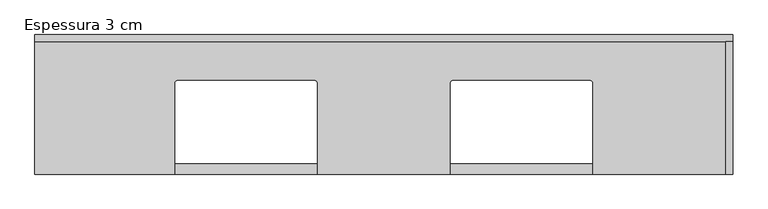
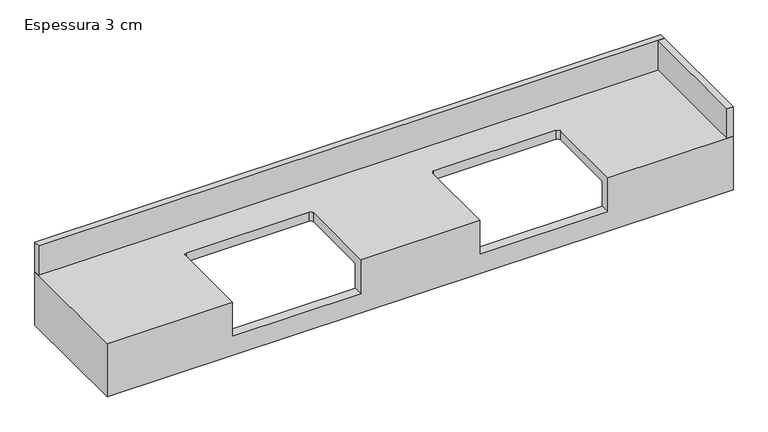
"""IFC4 building model written with IfcOpenShell, lengths in millimetres: furniture geometry, CC_BANCADA BANHEIRO COM DUAS CUBAS_CANTO RETO : Espessura 3 cm."""

import ifcopenshell
import ifcopenshell.guid

model = None  # the IFC model being written
_history = None  # IfcOwnerHistory: only IFC2X3 demands one
_inside = {}  # id of a spatial element -> (the spatial element, [elements in it])
_under = {}  # id of a project, library or spatial element -> (it, [spatial elements below it])
_declared = {}  # id of a project -> (the project, [libraries it declares])
_typed = {}  # id of a type object -> (the type object, [elements of that type])
_made_of = {}  # id of a material, layer set ... -> (it, [elements and type objects made of it])


def new_model(schema):
    """Start an empty IFC model of exactly this schema.

    Asked for "IFC4X3", IfcOpenShell would pick the latest addendum, in which some entities
    have other attributes; the version numbers below select the first issue.
    IFC2X3 requires an IfcOwnerHistory on every rooted entity: one is made here for all.
    """
    global model, _history
    if schema == "IFC4X3":
        model = ifcopenshell.file(schema_version=(4, 3, 0, 0))
    else:
        model = ifcopenshell.file(schema=schema)
    _inside.clear()
    _under.clear()
    _declared.clear()
    _typed.clear()
    _made_of.clear()
    _history = None
    if model.schema == "IFC2X3":
        org = make("IfcOrganization", Name="unknown")
        user = make(
            "IfcPersonAndOrganization",
            ThePerson=make("IfcPerson", FamilyName="unknown"),
            TheOrganization=org,
        )
        app = make(
            "IfcApplication",
            ApplicationDeveloper=org,
            Version="unknown",
            ApplicationFullName="unknown",
            ApplicationIdentifier="unknown",
        )
        _history = make(
            "IfcOwnerHistory",
            OwningUser=user,
            OwningApplication=app,
            ChangeAction="ADDED",
            CreationDate=0,
        )
    return model


def make(cls, **values):
    """One entity of the class cls with the attributes given. An attribute that is None is left unset."""
    return model.create_entity(
        cls, **{name: value for name, value in values.items() if value is not None}
    )


def rooted(cls, **values):
    """An entity with a GlobalId (a new one), such as an element, a storey or a relation."""
    return make(cls, GlobalId=ifcopenshell.guid.new(), OwnerHistory=_history, **values)


def si_unit(unit_type, name, prefix=None):
    """IfcSIUnit, for example si_unit("LENGTHUNIT", "METRE", prefix="MILLI")."""
    return make("IfcSIUnit", UnitType=unit_type, Prefix=prefix, Name=name)


def assignment(units):
    """IfcUnitAssignment: the units of a project."""
    return None if units is None else make("IfcUnitAssignment", Units=units)


def point(xyz):
    """IfcCartesianPoint."""
    return None if xyz is None else make("IfcCartesianPoint", Coordinates=xyz)


def direction(xyz):
    """IfcDirection."""
    return None if xyz is None else make("IfcDirection", DirectionRatios=xyz)


def frame(location, z_axis=None, x_axis=None):
    """IfcAxis2Placement3D, a coordinate frame: its origin and axes. An axis left out is left unset."""
    return make(
        "IfcAxis2Placement3D",
        Location=point(location),
        Axis=direction(z_axis),
        RefDirection=direction(x_axis),
    )


def origin():
    """The frame at (0, 0, 0) with its axes left unset."""
    return frame((0.0, 0.0, 0.0))


def place(relative_to, where):
    """IfcLocalPlacement: puts the frame where relative to a parent placement (None: the world)."""
    return make(
        "IfcLocalPlacement", PlacementRelTo=relative_to, RelativePlacement=where
    )


def context(
    kind, dimensions, precision=None, world=None, true_north=None, identifier=None
):
    """IfcGeometricRepresentationContext, for example the 3D "Model" context."""
    return make(
        "IfcGeometricRepresentationContext",
        ContextIdentifier=identifier,
        ContextType=kind,
        CoordinateSpaceDimension=dimensions,
        Precision=precision,
        WorldCoordinateSystem=world,
        TrueNorth=true_north,
    )


def project(units=None, contexts=None):
    """IfcProject with its units and contexts."""
    return rooted(
        "IfcProject",
        Name="project",
        RepresentationContexts=contexts,
        UnitsInContext=assignment(units),
    )


def spatial(cls, under=None, at=None, **own):
    """A site, building, storey or space (cls), placed at a placement, below another one or the project."""
    s = rooted(cls, ObjectPlacement=at, **own)
    if under is not None:
        _under.setdefault(under.id(), (under, []))[1].append(s)
    return s


def polyline(points):
    """IfcPolyline through the points."""
    return make("IfcPolyline", Points=[point(p) for p in points])


def circle_curve(where, radius):
    """IfcCircle in the frame where."""
    return make("IfcCircle", Position=where, Radius=radius)


def outline(outer, holes=None, kind="AREA"):
    """IfcArbitraryClosedProfileDef: a profile drawn as a closed curve; with holes, ...WithVoids."""
    if holes is None:
        return make("IfcArbitraryClosedProfileDef", ProfileType=kind, OuterCurve=outer)
    return make(
        "IfcArbitraryProfileDefWithVoids",
        ProfileType=kind,
        OuterCurve=outer,
        InnerCurves=holes,
    )


def extrude(swept, where, along, depth):
    """IfcExtrudedAreaSolid: the profile swept, set in the frame where, extruded along a direction by depth."""
    return make(
        "IfcExtrudedAreaSolid",
        SweptArea=swept,
        Position=where,
        ExtrudedDirection=direction(along),
        Depth=depth,
    )


def shape(context_of_items, identifier, shape_type, items):
    """IfcShapeRepresentation: the items that make up one representation, for example the "Body"."""
    return make(
        "IfcShapeRepresentation",
        ContextOfItems=context_of_items,
        RepresentationIdentifier=identifier,
        RepresentationType=shape_type,
        Items=items,
    )


def source(mapping_origin, context_of_items, identifier, shape_type, items):
    """IfcRepresentationMap: a shape defined once, which mapped items show again and again."""
    return make(
        "IfcRepresentationMap",
        MappingOrigin=mapping_origin,
        MappedRepresentation=shape(context_of_items, identifier, shape_type, items),
    )


def transform(
    local_origin,
    x_axis=None,
    y_axis=None,
    z_axis=None,
    scale=None,
    scale2=None,
    scale3=None,
    uniform=True,
):
    """IfcCartesianTransformationOperator3D, or its non-uniform kind. x_axis, y_axis, z_axis: its Axis1, 2, 3."""
    if uniform:
        return make(
            "IfcCartesianTransformationOperator3D",
            Axis1=direction(x_axis),
            Axis2=direction(y_axis),
            LocalOrigin=point(local_origin),
            Scale=scale,
            Axis3=direction(z_axis),
        )
    return make(
        "IfcCartesianTransformationOperator3DnonUniform",
        Axis1=direction(x_axis),
        Axis2=direction(y_axis),
        LocalOrigin=point(local_origin),
        Scale=scale,
        Axis3=direction(z_axis),
        Scale2=scale2,
        Scale3=scale3,
    )


def mapped(mapping_source, mapping_target):
    """IfcMappedItem: shows the shape of a source again, moved by a transform."""
    return make(
        "IfcMappedItem", MappingSource=mapping_source, MappingTarget=mapping_target
    )


def made_of(thing, what):
    """Note that an element or type object is made of a material, layer set ...; save() writes the relation."""
    if what is not None:
        _made_of.setdefault(what.id(), (what, []))[1].append(thing)
    return thing


def element(
    cls,
    number,
    at=None,
    inside=None,
    cuts=None,
    type_object=None,
    material=None,
    context=None,
    identifier="Body",
    shape_type=None,
    held_by="IfcProductDefinitionShape",
    body=None,
    shapes=None,
    **own,
):
    """One element of the class cls, such as IfcWall. Its Tag is "e" and its number.

    at: its placement. inside: the storey or other place that contains it. cuts: it is an
    opening in that element (IfcRelVoidsElement). A single representation is given by context,
    identifier, shape_type and body (its items); several are given by shapes. held_by: the class
    of the entity that holds the representations. save() writes the other relations.
    """
    e = rooted(cls, Tag="e%d" % number, ObjectPlacement=at, **own)
    if body is not None:
        shapes = [shape(context, identifier, shape_type, body)]
    if shapes is not None:
        e.Representation = make(held_by, Representations=shapes)
    if inside is not None:
        _inside.setdefault(inside.id(), (inside, []))[1].append(e)
    if cuts is not None:
        rooted(
            "IfcRelVoidsElement", RelatingBuildingElement=cuts, RelatedOpeningElement=e
        )
    if type_object is not None:
        _typed.setdefault(type_object.id(), (type_object, []))[1].append(e)
    return made_of(e, material)


def aggregate(whole, parts):
    """IfcRelAggregates: a whole, such as a stair, and the parts it consists of."""
    return rooted("IfcRelAggregates", RelatingObject=whole, RelatedObjects=parts)


def save(model, path):
    """Write the relations noted so far, then the file.

    IfcRelAggregates (storeys below a building ...), IfcRelContainedInSpatialStructure (elements
    in a storey), IfcRelDefinesByType, IfcRelAssociatesMaterial and IfcRelDeclares: one each for
    every whole, place, type object, material and project.
    """
    for whole, parts in _under.values():
        aggregate(whole, parts)
    for where, things in _inside.values():
        rooted(
            "IfcRelContainedInSpatialStructure",
            RelatedElements=things,
            RelatingStructure=where,
        )
    for kind, things in _typed.values():
        rooted("IfcRelDefinesByType", RelatedObjects=things, RelatingType=kind)
    for what, things in _made_of.values():
        rooted("IfcRelAssociatesMaterial", RelatedObjects=things, RelatingMaterial=what)
    for by, libraries in _declared.values():
        rooted("IfcRelDeclares", RelatingContext=by, RelatedDefinitions=libraries)
    model.write(path)


def plane_surface(at):
    """IfcPlane: the flat surface through the origin of the frame at, square to its z axis."""
    return make("IfcPlane", Position=at)


def revolved_surface(curve, axis_point, axis_direction):
    """IfcSurfaceOfRevolution: the curve turned about the line through axis_point along axis_direction."""
    return make(
        "IfcSurfaceOfRevolution",
        SweptCurve=make("IfcArbitraryOpenProfileDef", ProfileType="CURVE", Curve=curve),
        AxisPosition=make("IfcAxis1Placement", Location=point(axis_point), Axis=direction(axis_direction)),
    )


def advanced_brep(points, edges, surfaces, faces):
    """IfcAdvancedBrep: a solid bounded by faces that lie on surfaces and meet in shared edges.

    An edge is (start, end): straight between two places in points (the first is 0);
    or (start, end, curve); or (start, end, curve, False) where it runs against its curve.
    A face is (place in surfaces, loops), or (place, loops, False) where it looks against
    its surface's normal. A loop lists edges by number (the first is 1), with a minus sign
    where the edge is run from its end to its start. The first loop is the outer one.
    """
    corners = [point(p) for p in points]
    vertices = [make("IfcVertexPoint", VertexGeometry=c) for c in corners]
    made = []
    for start, end, *more in edges:
        made.append(
            make(
                "IfcEdgeCurve",
                EdgeStart=vertices[start],
                EdgeEnd=vertices[end],
                EdgeGeometry=more[0] if more else make("IfcPolyline", Points=[corners[start], corners[end]]),
                SameSense=more[1] if len(more) > 1 else True,
            )
        )
    hull = []
    for where, loops, *sense in faces:
        bounds = []
        for j, loop in enumerate(loops):
            ring = [make("IfcOrientedEdge", EdgeElement=made[abs(k) - 1], Orientation=k > 0) for k in loop]
            bounds.append(
                make(
                    "IfcFaceOuterBound" if j == 0 else "IfcFaceBound",
                    Bound=make("IfcEdgeLoop", EdgeList=ring),
                    Orientation=True,
                )
            )
        hull.append(make("IfcAdvancedFace", Bounds=bounds, FaceSurface=surfaces[where], SameSense=sense[0] if sense else True))
    return make("IfcAdvancedBrep", Outer=make("IfcClosedShell", CfsFaces=hull))


def espessura_3_cm_7ff6149e(model_context):
    return source(origin(), model_context, "Body", "SolidModel", [
        advanced_brep(
        [(750.0, 300.0, 860.0), (-1250.0, 300.0, 860.0), (-1250.0, -100.0, 860.0), (-850.0, -100.0, 860.0), (-850.0, 160.0, 860.0), (-840.0, 170.0, 860.0), (-450.0, 170.0, 860.0), (-440.0, 160.0, 860.0), (-440.0, -100.0, 860.0), (-60.0, -100.0, 860.0), (-60.0, 160.0, 860.0), (-50.0, 170.0, 860.0), (340.0, 170.0, 860.0), (350.0, 160.0, 860.0), (350.0, -100.0, 860.0), (750.0, -100.0, 860.0), (750.0, 300.0, 680.0), (720.0, 300.0, 680.0), (720.0, 300.0, 830.0), (-1220.0, 300.0, 830.0), (-1220.0, 300.0, 680.0), (-1250.0, 300.0, 680.0), (-1250.0, -100.0, 680.0), (750.0, -100.0, 680.0), (350.0, -100.0, 745.0), (-60.0, -100.0, 745.0), (-440.0, -100.0, 745.0), (-850.0, -100.0, 745.0), (720.0, -70.0, 830.0), (350.0, -70.0, 830.0), (350.0, 160.0, 830.0), (340.0, 170.0, 830.0), (-50.0, 170.0, 830.0), (-60.0, 160.0, 830.0), (-60.0, -70.0, 830.0), (-440.0, -70.0, 830.0), (-440.0, 160.0, 830.0), (-450.0, 170.0, 830.0), (-840.0, 170.0, 830.0), (-850.0, 160.0, 830.0), (-850.0, -70.0, 830.0), (-1220.0, -70.0, 830.0), (-1220.0, -70.0, 680.0), (-850.0, -70.0, 745.0), (-440.0, -70.0, 745.0), (-60.0, -70.0, 745.0), (350.0, -70.0, 745.0), (720.0, -70.0, 680.0)],
        [
            (0, 1),
            (1, 2),
            (2, 3),
            (3, 4),
            (4, 5, circle_curve(frame((-840.0, 160.0, 860.0), z_axis=(0.0, 0.0, -1.0), x_axis=(0.0, 1.0, 0.0)), 10.0)),
            (5, 6),
            (6, 7, circle_curve(frame((-450.0, 160.0, 860.0), z_axis=(0.0, 0.0, -1.0), x_axis=(0.0, 1.0, 0.0)), 10.0)),
            (7, 8),
            (8, 9),
            (9, 10),
            (10, 11, circle_curve(frame((-50.0, 160.0, 860.0), z_axis=(0.0, 0.0, -1.0), x_axis=(0.0, 1.0, 0.0)), 10.0)),
            (11, 12),
            (12, 13, circle_curve(frame((340.0, 160.0, 860.0), z_axis=(0.0, 0.0, -1.0), x_axis=(0.0, 1.0, 0.0)), 10.0)),
            (13, 14),
            (14, 15),
            (15, 0),
            (0, 16),
            (16, 17),
            (17, 18),
            (18, 19),
            (19, 20),
            (20, 21),
            (21, 1),
            (21, 22),
            (22, 2),
            (22, 23),
            (23, 15),
            (14, 24),
            (24, 25),
            (25, 9),
            (8, 26),
            (26, 27),
            (27, 3),
            (23, 16),
            (18, 28),
            (28, 29),
            (29, 30),
            (30, 31, circle_curve(frame((340.0, 160.0, 830.0), z_axis=(0.0, 0.0, 1.0), x_axis=(0.0, 1.0, 0.0)), 10.0)),
            (31, 32),
            (32, 33, circle_curve(frame((-50.0, 160.0, 830.0), z_axis=(0.0, 0.0, 1.0), x_axis=(0.0, 1.0, 0.0)), 10.0)),
            (33, 34),
            (34, 35),
            (35, 36),
            (36, 37, circle_curve(frame((-450.0, 160.0, 830.0), z_axis=(0.0, 0.0, 1.0), x_axis=(0.0, 1.0, 0.0)), 10.0)),
            (37, 38),
            (38, 39, circle_curve(frame((-840.0, 160.0, 830.0), z_axis=(0.0, 0.0, 1.0), x_axis=(0.0, 1.0, 0.0)), 10.0)),
            (39, 40),
            (40, 41),
            (41, 19),
            (41, 42),
            (42, 20),
            (40, 43),
            (43, 44),
            (44, 35),
            (34, 45),
            (45, 46),
            (46, 29),
            (28, 47),
            (47, 42),
            (17, 47),
            (5, 38),
            (37, 6),
            (26, 44),
            (43, 27),
            (4, 39),
            (7, 36),
            (24, 46),
            (45, 25),
            (11, 32),
            (31, 12),
            (10, 33),
            (13, 30),
        ],
        [
            plane_surface(frame((-1250.0, 300.0, 860.0), z_axis=(0.0, 0.0, 1.0), x_axis=(-1.0, 0.0, 0.0))),
            plane_surface(frame((750.0, 300.0, 860.0), z_axis=(0.0, 1.0, 0.0), x_axis=(0.0, 0.0, -1.0))),
            plane_surface(frame((-1250.0, 300.0, 860.0), z_axis=(-1.0, 0.0, 0.0), x_axis=(0.0, 0.0, -1.0))),
            plane_surface(frame((-1250.0, -100.0, 860.0), z_axis=(0.0, -1.0, 0.0), x_axis=(0.0, 0.0, -1.0))),
            plane_surface(frame((750.0, -100.0, 860.0), z_axis=(1.0, 0.0, 0.0), x_axis=(0.0, 0.0, -1.0))),
            plane_surface(frame((-1220.0, 300.0, 830.0), z_axis=(0.0, 0.0, -1.0), x_axis=(-1.0, 0.0, 0.0))),
            plane_surface(frame((-1220.0, 300.0, 830.0), z_axis=(1.0, 0.0, 0.0), x_axis=(0.0, 0.0, -1.0))),
            plane_surface(frame((-1220.0, -70.0, 830.0), z_axis=(0.0, 1.0, 0.0), x_axis=(0.0, 0.0, -1.0))),
            plane_surface(frame((720.0, -70.0, 830.0), z_axis=(-1.0, 0.0, 0.0), x_axis=(0.0, 0.0, -1.0))),
            plane_surface(frame((750.0, -100.0, 680.0), z_axis=(0.0, 0.0, -1.0), x_axis=(0.0, 1.0, 0.0))),
            plane_surface(frame((-840.0, 170.0, 745.0), z_axis=(0.0, -1.0, 0.0), x_axis=(0.0, 0.0, 1.0))),
            plane_surface(frame((-450.0, 170.0, 745.0), z_axis=(0.0, 0.0, 1.0), x_axis=(1.0, 0.0, 0.0))),
            revolved_surface(polyline([(-840.0, 170.0, 830.0), (-840.0, 170.0, 860.0)]), (-840.0, 160.0, 900.0), (0.0, 0.0, -1.0)),
            plane_surface(frame((-850.0, -230.0, 745.0), z_axis=(1.0, 0.0, 0.0), x_axis=(0.0, 0.0, 1.0))),
            plane_surface(frame((-440.0, 160.0, 745.0), z_axis=(-1.0, 0.0, 0.0), x_axis=(0.0, 0.0, 1.0))),
            revolved_surface(polyline([(-450.0, 170.0, 830.0), (-450.0, 170.0, 860.0)]), (-450.0, 160.0, 900.0), (0.0, 0.0, -1.0)),
            plane_surface(frame((340.0, 170.0, 745.0), z_axis=(0.0, 0.0, 1.0), x_axis=(1.0, 0.0, 0.0))),
            plane_surface(frame((-50.0, 170.0, 745.0), z_axis=(0.0, -1.0, 0.0), x_axis=(0.0, 0.0, 1.0))),
            revolved_surface(polyline([(-50.0, 170.0, 830.0), (-50.0, 170.0, 860.0)]), (-50.0, 160.0, 900.0), (0.0, 0.0, -1.0)),
            plane_surface(frame((-60.0, -230.0, 745.0), z_axis=(1.0, 0.0, 0.0), x_axis=(0.0, 0.0, 1.0))),
            plane_surface(frame((350.0, 160.0, 745.0), z_axis=(-1.0, 0.0, 0.0), x_axis=(0.0, 0.0, 1.0))),
            revolved_surface(polyline([(340.0, 170.0, 830.0), (340.0, 170.0, 860.0)]), (340.0, 160.0, 900.0), (0.0, 0.0, -1.0)),
        ],
        [
            (0, [[1, 2, 3, 4, 5, 6, 7, 8, 9, 10, 11, 12, 13, 14, 15, 16]]),
            (1, [[-1, 17, 18, 19, 20, 21, 22, 23]]),
            (2, [[-2, -23, 24, 25]]),
            (3, [[-3, -25, 26, 27, -15, 28, 29, 30, -9, 31, 32, 33]]),
            (4, [[-16, -27, 34, -17]]),
            (5, [[35, 36, 37, 38, 39, 40, 41, 42, 43, 44, 45, 46, 47, 48, 49, -20]]),
            (6, [[-49, 50, 51, -21]]),
            (7, [[-48, 52, 53, 54, -42, 55, 56, 57, -36, 58, 59, -50]]),
            (8, [[-35, -19, 60, -58]]),
            (9, [[-18, -34, -26, -24, -22, -51, -59, -60]]),
            (10, [[-6, 61, -45, 62]]),
            (11, [[-32, 63, -53, 64]]),
            (12, [[-5, 65, -46, -61]]),
            (13, [[-4, -33, -64, -52, -47, -65]]),
            (14, [[-8, 66, -43, -54, -63, -31]]),
            (15, [[-7, -62, -44, -66]]),
            (16, [[-29, 67, -56, 68]]),
            (17, [[-12, 69, -39, 70]]),
            (18, [[-11, 71, -40, -69]]),
            (19, [[-10, -30, -68, -55, -41, -71]]),
            (20, [[-14, 72, -37, -57, -67, -28]]),
            (21, [[-13, -70, -38, -72]]),
        ],
    ),
        extrude(outline(polyline([(730.0, 280.0), (750.0, 280.0), (750.0, -100.0), (730.0, -100.0), (730.0, 280.0)])), frame((0.0, 0.0, 860.0), z_axis=(0.0, 0.0, 1.0), x_axis=(1.0, 0.0, 0.0)), (0.0, 0.0, 1.0), 100.0),
        extrude(outline(polyline([(750.0, 300.0), (750.0, 280.0), (-1250.0, 280.0), (-1250.0, 300.0), (750.0, 300.0)])), frame((0.0, 0.0, 860.0), z_axis=(0.0, 0.0, 1.0), x_axis=(1.0, 0.0, 0.0)), (0.0, 0.0, 1.0), 100.0),
    ])


if __name__ == "__main__":
    model = new_model("IFC4")
    model_context = context("Model", 3, world=origin())
    ifc_project = project(units=[si_unit("LENGTHUNIT", "METRE", prefix="MILLI")], contexts=[model_context])
    site = spatial("IfcSite", under=ifc_project)
    building = spatial("IfcBuilding", under=site)
    placement = place(None, origin())
    espessura_3_cm_shape = espessura_3_cm_7ff6149e(model_context)
    element("IfcFurniture", 1, ObjectType="CC_BANCADA BANHEIRO COM DUAS CUBAS_CANTO RETO : Espessura 3 cm", at=placement, inside=building, context=model_context, shape_type="MappedRepresentation", body=[
        mapped(espessura_3_cm_shape, transform((0.0, 0.0, 0.0), x_axis=(1.0, 0.0, 0.0), y_axis=(0.0, 1.0, 0.0), z_axis=(0.0, 0.0, 1.0))),
    ])
    save(model, "model.ifc")

# Revit data of these elements
# Type "CC_BANCADA BANHEIRO COM DUAS CUBAS_CANTO RETO : Espessura 3 cm"
#   Uso HS [instance default] = ""
#   h TESTEIRA AUX [instance default] = 0.15 m
#   Altura testeira [instance default] = 0.15 m
#   Altura rodapia [instance default] = 0.10 m
#   Espessura rodapia [instance default] = 0.02 m
#   Prof/2 [instance default] = 0.20 m
#   Offset cuba direita [instance default] = 0.40 m
#   Offset cuba esquerda [instance default] = 0.40 m
#   Depth [instance default] = 2.00 m
#   Width [instance default] = 0.40 m
#   Espessura bancada = 0.03 m
#   Comprimento [instance default] = 2.00 m
#   Height [instance default] = 0.86 m
#   Testeira [instance default] = yes
#   Rodapia fundo [instance default] = no
#   Rodapia esquerda [instance default] = no
#   Rodapia direita [instance default] = no
#   Material porta-toalha [instance default] = .CROMADO
#   Material hidráulico [instance default] = .CROMADO
#   Material cuba [instance default] = .PORCELANA BRANCA
#   Material bancada [instance default] = .GRANITO_BRANCO_ITAUNAS
#   Assembly Code = ""
# Element 1 (IfcFurniture, "CC_BANCADA BANHEIRO COM DUAS CUBAS_CANTO RETO : Espessura 3 cm")
#   Uso HS = "SUÍTE MASTER"
#   Rodapia fundo = yes
#   Rodapia direita = yes
#   Materials on its faces: ".GRANITO_BRANCO_ITAUNAS"
# Materials
#   ".CROMADO": class "CC_METAIS", colour RGB 211 223 226, transparency 0, Cost = 0
#   ".PORCELANA BRANCA": class "CC_PORCELANA", colour RGB 230 230 230, transparency 0, Cost = 0
#   ".GRANITO_BRANCO_ITAUNAS": class ".CC_PEDRA REVEST.", colour RGB 202 195 174, transparency 0, Description = "Revestimento em granito", Cost = 0
